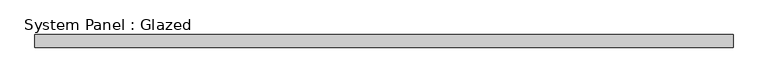
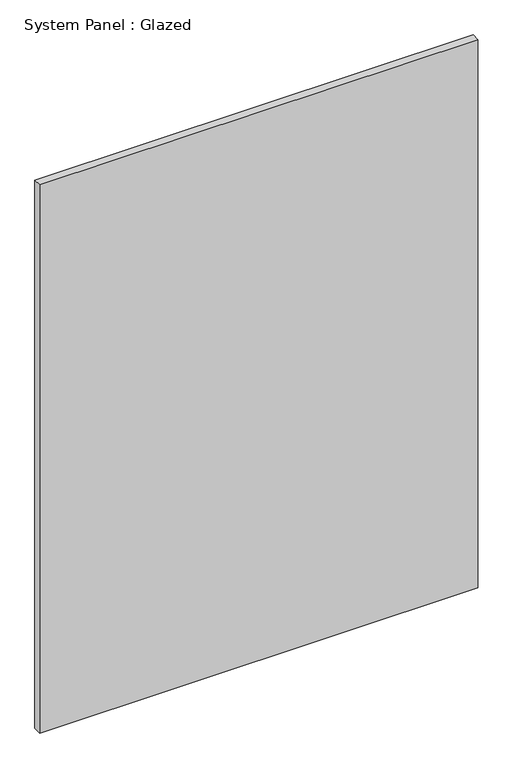
"""IFC4 building model written with IfcOpenShell, lengths in millimetres: plate geometry, System Panel : Glazed."""

from ifc_helpers import new_model, si_unit, origin, origin_with_axes, place, context, project, spatial, polyline, outline, extrude, source, transform, mapped, element, save


def system_panel_glazed_52881cd9(model_context):
    return source(origin(), model_context, "Body", "SweptSolid", [
        extrude(outline(polyline([(669.9999999, 24.5), (-669.9999999, 24.5), (-669.9999999, 49.5), (669.9999999, 49.5), (669.9999999, 24.5)])), origin_with_axes(), (0.0, 0.0, 1.0), 1772.3836314),
    ])


if __name__ == "__main__":
    model = new_model("IFC4")
    model_context = context("Model", 3, world=origin())
    ifc_project = project(units=[si_unit("LENGTHUNIT", "METRE", prefix="MILLI")], contexts=[model_context])
    site = spatial("IfcSite", under=ifc_project)
    building = spatial("IfcBuilding", under=site)
    placement = place(None, origin())
    system_panel_glazed_shape = system_panel_glazed_52881cd9(model_context)
    element("IfcPlate", 1, ObjectType="System Panel : Glazed", at=placement, inside=building, context=model_context, shape_type="MappedRepresentation", body=[
        mapped(system_panel_glazed_shape, transform((0.0, 0.0, 0.0), x_axis=(1.0, 0.0, 0.0), y_axis=(0.0, 1.0, 0.0), z_axis=(0.0, 0.0, 1.0))),
    ])
    save(model, "model.ifc")

# Revit data of these elements
# Element 1 (IfcPlate, "System Panel : Glazed")
#   Materials on its faces: "Glass"
# Materials
#   "Glass": class "Glass", colour RGB 218 227 224, transparency 0.85, Description = "Soda Lime Glass", Cost = 0
